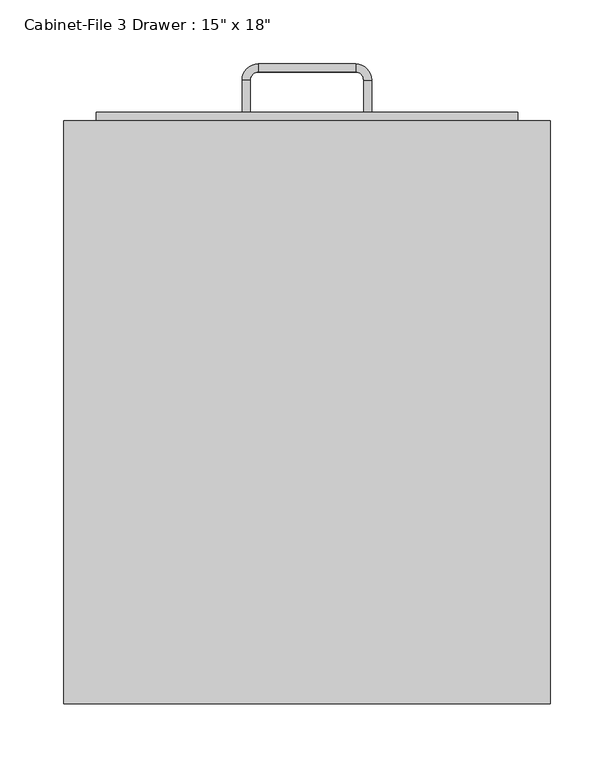
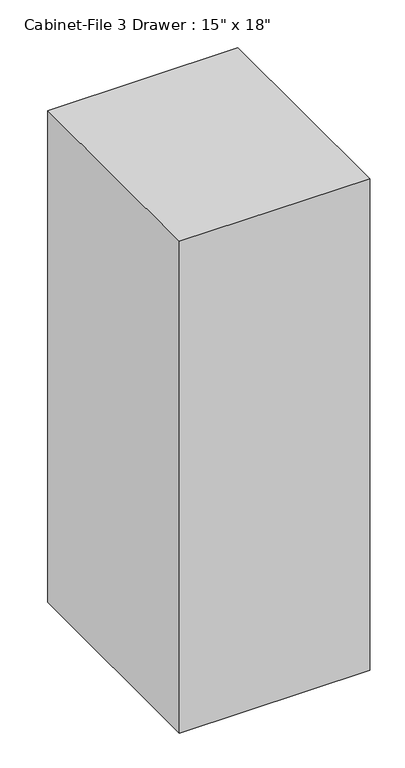
"""IFC4 building model written with IfcOpenShell, lengths in millimetres: furniture geometry."""

import ifcopenshell
import ifcopenshell.guid

model = None  # the IFC model being written
_history = None  # IfcOwnerHistory: only IFC2X3 demands one
_inside = {}  # id of a spatial element -> (the spatial element, [elements in it])
_under = {}  # id of a project, library or spatial element -> (it, [spatial elements below it])
_declared = {}  # id of a project -> (the project, [libraries it declares])
_typed = {}  # id of a type object -> (the type object, [elements of that type])
_made_of = {}  # id of a material, layer set ... -> (it, [elements and type objects made of it])


def new_model(schema):
    """Start an empty IFC model of exactly this schema.

    Asked for "IFC4X3", IfcOpenShell would pick the latest addendum, in which some entities
    have other attributes; the version numbers below select the first issue.
    IFC2X3 requires an IfcOwnerHistory on every rooted entity: one is made here for all.
    """
    global model, _history
    if schema == "IFC4X3":
        model = ifcopenshell.file(schema_version=(4, 3, 0, 0))
    else:
        model = ifcopenshell.file(schema=schema)
    _inside.clear()
    _under.clear()
    _declared.clear()
    _typed.clear()
    _made_of.clear()
    _history = None
    if model.schema == "IFC2X3":
        org = make("IfcOrganization", Name="unknown")
        user = make(
            "IfcPersonAndOrganization",
            ThePerson=make("IfcPerson", FamilyName="unknown"),
            TheOrganization=org,
        )
        app = make(
            "IfcApplication",
            ApplicationDeveloper=org,
            Version="unknown",
            ApplicationFullName="unknown",
            ApplicationIdentifier="unknown",
        )
        _history = make(
            "IfcOwnerHistory",
            OwningUser=user,
            OwningApplication=app,
            ChangeAction="ADDED",
            CreationDate=0,
        )
    return model


def make(cls, **values):
    """One entity of the class cls with the attributes given. An attribute that is None is left unset."""
    return model.create_entity(
        cls, **{name: value for name, value in values.items() if value is not None}
    )


def rooted(cls, **values):
    """An entity with a GlobalId (a new one), such as an element, a storey or a relation."""
    return make(cls, GlobalId=ifcopenshell.guid.new(), OwnerHistory=_history, **values)


def si_unit(unit_type, name, prefix=None):
    """IfcSIUnit, for example si_unit("LENGTHUNIT", "METRE", prefix="MILLI")."""
    return make("IfcSIUnit", UnitType=unit_type, Prefix=prefix, Name=name)


def assignment(units):
    """IfcUnitAssignment: the units of a project."""
    return None if units is None else make("IfcUnitAssignment", Units=units)


def point(xyz):
    """IfcCartesianPoint."""
    return None if xyz is None else make("IfcCartesianPoint", Coordinates=xyz)


def direction(xyz):
    """IfcDirection."""
    return None if xyz is None else make("IfcDirection", DirectionRatios=xyz)


def frame(location, z_axis=None, x_axis=None):
    """IfcAxis2Placement3D, a coordinate frame: its origin and axes. An axis left out is left unset."""
    return make(
        "IfcAxis2Placement3D",
        Location=point(location),
        Axis=direction(z_axis),
        RefDirection=direction(x_axis),
    )


def origin():
    """The frame at (0, 0, 0) with its axes left unset."""
    return frame((0.0, 0.0, 0.0))


def origin_with_axes():
    """The frame at (0, 0, 0) with the z axis (0, 0, 1) and the x axis (1, 0, 0) written out."""
    return frame((0.0, 0.0, 0.0), z_axis=(0.0, 0.0, 1.0), x_axis=(1.0, 0.0, 0.0))


def place(relative_to, where):
    """IfcLocalPlacement: puts the frame where relative to a parent placement (None: the world)."""
    return make(
        "IfcLocalPlacement", PlacementRelTo=relative_to, RelativePlacement=where
    )


def context(
    kind, dimensions, precision=None, world=None, true_north=None, identifier=None
):
    """IfcGeometricRepresentationContext, for example the 3D "Model" context."""
    return make(
        "IfcGeometricRepresentationContext",
        ContextIdentifier=identifier,
        ContextType=kind,
        CoordinateSpaceDimension=dimensions,
        Precision=precision,
        WorldCoordinateSystem=world,
        TrueNorth=true_north,
    )


def project(units=None, contexts=None):
    """IfcProject with its units and contexts."""
    return rooted(
        "IfcProject",
        Name="project",
        RepresentationContexts=contexts,
        UnitsInContext=assignment(units),
    )


def spatial(cls, under=None, at=None, **own):
    """A site, building, storey or space (cls), placed at a placement, below another one or the project."""
    s = rooted(cls, ObjectPlacement=at, **own)
    if under is not None:
        _under.setdefault(under.id(), (under, []))[1].append(s)
    return s


def polyline(points):
    """IfcPolyline through the points."""
    return make("IfcPolyline", Points=[point(p) for p in points])


def circle_curve(where, radius):
    """IfcCircle in the frame where."""
    return make("IfcCircle", Position=where, Radius=radius)


def outline(outer, holes=None, kind="AREA"):
    """IfcArbitraryClosedProfileDef: a profile drawn as a closed curve; with holes, ...WithVoids."""
    if holes is None:
        return make("IfcArbitraryClosedProfileDef", ProfileType=kind, OuterCurve=outer)
    return make(
        "IfcArbitraryProfileDefWithVoids",
        ProfileType=kind,
        OuterCurve=outer,
        InnerCurves=holes,
    )


def extrude(swept, where, along, depth):
    """IfcExtrudedAreaSolid: the profile swept, set in the frame where, extruded along a direction by depth."""
    return make(
        "IfcExtrudedAreaSolid",
        SweptArea=swept,
        Position=where,
        ExtrudedDirection=direction(along),
        Depth=depth,
    )


def shape(context_of_items, identifier, shape_type, items):
    """IfcShapeRepresentation: the items that make up one representation, for example the "Body"."""
    return make(
        "IfcShapeRepresentation",
        ContextOfItems=context_of_items,
        RepresentationIdentifier=identifier,
        RepresentationType=shape_type,
        Items=items,
    )


def source(mapping_origin, context_of_items, identifier, shape_type, items):
    """IfcRepresentationMap: a shape defined once, which mapped items show again and again."""
    return make(
        "IfcRepresentationMap",
        MappingOrigin=mapping_origin,
        MappedRepresentation=shape(context_of_items, identifier, shape_type, items),
    )


def transform(
    local_origin,
    x_axis=None,
    y_axis=None,
    z_axis=None,
    scale=None,
    scale2=None,
    scale3=None,
    uniform=True,
):
    """IfcCartesianTransformationOperator3D, or its non-uniform kind. x_axis, y_axis, z_axis: its Axis1, 2, 3."""
    if uniform:
        return make(
            "IfcCartesianTransformationOperator3D",
            Axis1=direction(x_axis),
            Axis2=direction(y_axis),
            LocalOrigin=point(local_origin),
            Scale=scale,
            Axis3=direction(z_axis),
        )
    return make(
        "IfcCartesianTransformationOperator3DnonUniform",
        Axis1=direction(x_axis),
        Axis2=direction(y_axis),
        LocalOrigin=point(local_origin),
        Scale=scale,
        Axis3=direction(z_axis),
        Scale2=scale2,
        Scale3=scale3,
    )


def mapped(mapping_source, mapping_target):
    """IfcMappedItem: shows the shape of a source again, moved by a transform."""
    return make(
        "IfcMappedItem", MappingSource=mapping_source, MappingTarget=mapping_target
    )


def made_of(thing, what):
    """Note that an element or type object is made of a material, layer set ...; save() writes the relation."""
    if what is not None:
        _made_of.setdefault(what.id(), (what, []))[1].append(thing)
    return thing


def element(
    cls,
    number,
    at=None,
    inside=None,
    cuts=None,
    type_object=None,
    material=None,
    context=None,
    identifier="Body",
    shape_type=None,
    held_by="IfcProductDefinitionShape",
    body=None,
    shapes=None,
    **own,
):
    """One element of the class cls, such as IfcWall. Its Tag is "e" and its number.

    at: its placement. inside: the storey or other place that contains it. cuts: it is an
    opening in that element (IfcRelVoidsElement). A single representation is given by context,
    identifier, shape_type and body (its items); several are given by shapes. held_by: the class
    of the entity that holds the representations. save() writes the other relations.
    """
    e = rooted(cls, Tag="e%d" % number, ObjectPlacement=at, **own)
    if body is not None:
        shapes = [shape(context, identifier, shape_type, body)]
    if shapes is not None:
        e.Representation = make(held_by, Representations=shapes)
    if inside is not None:
        _inside.setdefault(inside.id(), (inside, []))[1].append(e)
    if cuts is not None:
        rooted(
            "IfcRelVoidsElement", RelatingBuildingElement=cuts, RelatedOpeningElement=e
        )
    if type_object is not None:
        _typed.setdefault(type_object.id(), (type_object, []))[1].append(e)
    return made_of(e, material)


def aggregate(whole, parts):
    """IfcRelAggregates: a whole, such as a stair, and the parts it consists of."""
    return rooted("IfcRelAggregates", RelatingObject=whole, RelatedObjects=parts)


def save(model, path):
    """Write the relations noted so far, then the file.

    IfcRelAggregates (storeys below a building ...), IfcRelContainedInSpatialStructure (elements
    in a storey), IfcRelDefinesByType, IfcRelAssociatesMaterial and IfcRelDeclares: one each for
    every whole, place, type object, material and project.
    """
    for whole, parts in _under.values():
        aggregate(whole, parts)
    for where, things in _inside.values():
        rooted(
            "IfcRelContainedInSpatialStructure",
            RelatedElements=things,
            RelatingStructure=where,
        )
    for kind, things in _typed.values():
        rooted("IfcRelDefinesByType", RelatedObjects=things, RelatingType=kind)
    for what, things in _made_of.values():
        rooted("IfcRelAssociatesMaterial", RelatedObjects=things, RelatingMaterial=what)
    for by, libraries in _declared.values():
        rooted("IfcRelDeclares", RelatingContext=by, RelatedDefinitions=libraries)
    model.write(path)


def plane_surface(at):
    """IfcPlane: the flat surface through the origin of the frame at, square to its z axis."""
    return make("IfcPlane", Position=at)


def cylinder_surface(at, radius):
    """IfcCylindricalSurface: all points at the distance radius from the z axis of the frame at."""
    return make("IfcCylindricalSurface", Position=at, Radius=radius)


def revolved_surface(curve, axis_point, axis_direction):
    """IfcSurfaceOfRevolution: the curve turned about the line through axis_point along axis_direction."""
    return make(
        "IfcSurfaceOfRevolution",
        SweptCurve=make("IfcArbitraryOpenProfileDef", ProfileType="CURVE", Curve=curve),
        AxisPosition=make("IfcAxis1Placement", Location=point(axis_point), Axis=direction(axis_direction)),
    )


def advanced_brep(points, edges, surfaces, faces):
    """IfcAdvancedBrep: a solid bounded by faces that lie on surfaces and meet in shared edges.

    An edge is (start, end): straight between two places in points (the first is 0);
    or (start, end, curve); or (start, end, curve, False) where it runs against its curve.
    A face is (place in surfaces, loops), or (place, loops, False) where it looks against
    its surface's normal. A loop lists edges by number (the first is 1), with a minus sign
    where the edge is run from its end to its start. The first loop is the outer one.
    """
    corners = [point(p) for p in points]
    vertices = [make("IfcVertexPoint", VertexGeometry=c) for c in corners]
    made = []
    for start, end, *more in edges:
        made.append(
            make(
                "IfcEdgeCurve",
                EdgeStart=vertices[start],
                EdgeEnd=vertices[end],
                EdgeGeometry=more[0] if more else make("IfcPolyline", Points=[corners[start], corners[end]]),
                SameSense=more[1] if len(more) > 1 else True,
            )
        )
    hull = []
    for where, loops, *sense in faces:
        bounds = []
        for j, loop in enumerate(loops):
            ring = [make("IfcOrientedEdge", EdgeElement=made[abs(k) - 1], Orientation=k > 0) for k in loop]
            bounds.append(
                make(
                    "IfcFaceOuterBound" if j == 0 else "IfcFaceBound",
                    Bound=make("IfcEdgeLoop", EdgeList=ring),
                    Orientation=True,
                )
            )
        hull.append(make("IfcAdvancedFace", Bounds=bounds, FaceSurface=surfaces[where], SameSense=sense[0] if sense else True))
    return make("IfcAdvancedBrep", Outer=make("IfcClosedShell", CfsFaces=hull))


def furniture_48aa8ab9(model_context):
    return source(origin(), model_context, "Body", "SolidModel", [
        extrude(outline(polyline([(62.603553, -86.4656999), (-318.396447, -86.4656999), (-318.396447, 370.7343001), (62.603553, 370.7343001), (62.603553, -86.4656999)])), origin_with_axes(), (0.0, 0.0, 1.0), 1041.4),
        extrude(outline(polyline([(37.203553, 377.0843001), (37.203553, 370.7343001), (-292.996447, 370.7343001), (-292.996447, 377.0843001), (37.203553, 377.0843001)])), frame((0.0, 0.0, 736.6), z_axis=(0.0, 0.0, 1.0), x_axis=(1.0, 0.0, 0.0)), (0.0, 0.0, 1.0), 279.4),
        extrude(outline(polyline([(37.203553, 377.0843001), (37.203553, 370.7343001), (-292.996447, 370.7343001), (-292.996447, 377.0843001), (37.203553, 377.0843001)])), frame((0.0, 0.0, 431.8), z_axis=(0.0, 0.0, 1.0), x_axis=(1.0, 0.0, 0.0)), (0.0, 0.0, 1.0), 279.4),
        extrude(outline(polyline([(37.203553, 377.0843001), (37.203553, 370.7343001), (-292.996447, 370.7343001), (-292.996447, 377.0843001), (37.203553, 377.0843001)])), frame((0.0, 0.0, 127.0), z_axis=(0.0, 0.0, 1.0), x_axis=(1.0, 0.0, 0.0)), (0.0, 0.0, 1.0), 279.4),
        advanced_brep(
        [(-172.346447, 377.0843001, 203.2), (-172.346447, 377.0843001, 215.9), (-178.696447, 377.0843001, 215.9), (-178.696447, 377.0843001, 203.2), (-178.696447, 402.4843001, 203.2), (-172.346447, 402.4843001, 203.2), (-178.696447, 402.4843001, 215.9), (-172.346447, 402.4843001, 215.9), (-165.996447, 415.1843001, 203.2), (-165.996447, 408.8343001, 203.2), (-165.996447, 415.1843001, 215.9), (-165.996447, 408.8343001, 215.9), (-89.796447, 415.1843001, 203.2), (-89.796447, 408.8343001, 203.2), (-89.796447, 415.1843001, 215.9), (-89.796447, 408.8343001, 215.9), (-77.096447, 402.4843001, 203.2), (-83.446447, 402.4843001, 203.2), (-77.096447, 402.4843001, 215.9), (-83.446447, 402.4843001, 215.9), (-83.446447, 377.0843001, 203.2), (-77.096447, 377.0843001, 203.2), (-77.096447, 377.0843001, 215.9), (-83.446447, 377.0843001, 215.9)],
        [
            (0, 1),
            (1, 2),
            (2, 3),
            (3, 0),
            (3, 4),
            (4, 5),
            (5, 0),
            (2, 6),
            (6, 4),
            (1, 7),
            (7, 6),
            (5, 7),
            (8, 9),
            (9, 5, circle_curve(frame((-165.996447, 402.4843001, 203.2), z_axis=(0.0, 0.0, 1.0), x_axis=(-1.0, 0.0, 0.0)), 6.35)),
            (4, 8, circle_curve(frame((-165.996447, 402.4843001, 203.2), z_axis=(0.0, 0.0, -1.0), x_axis=(-1.0, 0.0, 0.0)), 12.7)),
            (10, 8),
            (6, 10, circle_curve(frame((-165.996447, 402.4843001, 215.9), z_axis=(0.0, 0.0, -1.0), x_axis=(-1.0, 0.0, 0.0)), 12.7)),
            (11, 10),
            (7, 11, circle_curve(frame((-165.996447, 402.4843001, 215.9), z_axis=(0.0, 0.0, -1.0), x_axis=(-1.0, 0.0, 0.0)), 6.35)),
            (9, 11),
            (8, 12),
            (12, 13),
            (13, 9),
            (10, 14),
            (14, 12),
            (11, 15),
            (15, 14),
            (13, 15),
            (16, 17),
            (17, 13, circle_curve(frame((-89.796447, 402.4843001, 203.2), z_axis=(0.0, 0.0, 1.0), x_axis=(0.0, 1.0, 0.0)), 6.35)),
            (12, 16, circle_curve(frame((-89.796447, 402.4843001, 203.2), z_axis=(0.0, 0.0, -1.0), x_axis=(0.0, 1.0, 0.0)), 12.7)),
            (18, 16),
            (14, 18, circle_curve(frame((-89.796447, 402.4843001, 215.9), z_axis=(0.0, 0.0, -1.0), x_axis=(0.0, 1.0, 0.0)), 12.7)),
            (19, 18),
            (15, 19, circle_curve(frame((-89.796447, 402.4843001, 215.9), z_axis=(0.0, 0.0, -1.0), x_axis=(0.0, 1.0, 0.0)), 6.35)),
            (17, 19),
            (20, 21),
            (21, 22),
            (22, 23),
            (23, 20),
            (16, 21),
            (20, 17),
            (18, 22),
            (19, 23),
        ],
        [
            plane_surface(frame((-978.8216451, 377.0843001, 0.0), z_axis=(0.0, -1.0, 0.0), x_axis=(0.0, 0.0, -1.0))),
            plane_surface(frame((-172.346447, 377.0843001, 203.2), z_axis=(0.0, 0.0, -1.0), x_axis=(0.0, 1.0, 0.0))),
            plane_surface(frame((-178.696447, 377.0843001, 203.2), z_axis=(-1.0, 0.0, 0.0), x_axis=(0.0, 1.0, 0.0))),
            plane_surface(frame((-178.696447, 377.0843001, 215.9), z_axis=(0.0, 0.0, 1.0), x_axis=(0.0, 1.0, 0.0))),
            plane_surface(frame((-172.346447, 377.0843001, 215.9), z_axis=(1.0, 0.0, 0.0), x_axis=(0.0, 1.0, 0.0))),
            plane_surface(frame((-165.996447, 402.4843001, 203.2), z_axis=(0.0, 0.0, -1.0), x_axis=(-1.0, 0.0, 0.0))),
            cylinder_surface(frame((-165.996447, 402.4843001, 0.0), z_axis=(0.0, 0.0, 1.0), x_axis=(-1.0, 0.0, 0.0)), 12.7),
            plane_surface(frame((-165.996447, 402.4843001, 215.9), z_axis=(0.0, 0.0, 1.0), x_axis=(-1.0, 0.0, 0.0))),
            revolved_surface(polyline([(-172.34644699999998, 402.4843001, 215.9), (-172.34644699999998, 402.4843001, 203.2)]), (-165.996447, 402.4843001, 0.0), (0.0, 0.0, 1.0)),
            plane_surface(frame((-165.996447, 408.8343001, 203.2), z_axis=(0.0, 0.0, -1.0), x_axis=(1.0, 0.0, 0.0))),
            plane_surface(frame((-165.996447, 415.1843001, 203.2), z_axis=(0.0, 1.0, 0.0), x_axis=(1.0, 0.0, 0.0))),
            plane_surface(frame((-165.996447, 415.1843001, 215.9), z_axis=(0.0, 0.0, 1.0), x_axis=(1.0, 0.0, 0.0))),
            plane_surface(frame((-165.996447, 408.8343001, 215.9), z_axis=(0.0, -1.0, 0.0), x_axis=(1.0, 0.0, 0.0))),
            plane_surface(frame((-89.796447, 402.4843001, 203.2), z_axis=(0.0, 0.0, -1.0), x_axis=(0.0, 1.0, 0.0))),
            cylinder_surface(frame((-89.796447, 402.4843001, 0.0), z_axis=(0.0, 0.0, 1.0), x_axis=(0.0, 1.0, 0.0)), 12.7),
            plane_surface(frame((-89.796447, 402.4843001, 215.9), z_axis=(0.0, 0.0, 1.0), x_axis=(0.0, 1.0, 0.0))),
            revolved_surface(polyline([(-89.796447, 408.8343001, 215.9), (-89.796447, 408.8343001, 203.2)]), (-89.796447, 402.4843001, 0.0), (0.0, 0.0, 1.0)),
            plane_surface(frame((-877.2216451, 377.0843001, 0.0), z_axis=(0.0, -1.0, 0.0), x_axis=(0.0, 0.0, 1.0))),
            plane_surface(frame((-83.446447, 402.4843001, 203.2), z_axis=(0.0, 0.0, -1.0), x_axis=(0.0, -1.0, 0.0))),
            plane_surface(frame((-77.096447, 402.4843001, 203.2), z_axis=(1.0, 0.0, 0.0), x_axis=(0.0, -1.0, 0.0))),
            plane_surface(frame((-77.096447, 402.4843001, 215.9), z_axis=(0.0, 0.0, 1.0), x_axis=(0.0, -1.0, 0.0))),
            plane_surface(frame((-83.446447, 402.4843001, 215.9), z_axis=(-1.0, 0.0, 0.0), x_axis=(0.0, -1.0, 0.0))),
        ],
        [
            (0, [[1, 2, 3, 4]]),
            (1, [[5, 6, 7, -4]]),
            (2, [[8, 9, -5, -3]]),
            (3, [[10, 11, -8, -2]]),
            (4, [[-7, 12, -10, -1]]),
            (5, [[13, 14, -6, 15]]),
            (6, [[16, -15, -9, 17]]),
            (7, [[18, -17, -11, 19]]),
            (8, [[20, -19, -12, -14]]),
            (9, [[21, 22, 23, -13]]),
            (10, [[24, 25, -21, -16]]),
            (11, [[26, 27, -24, -18]]),
            (12, [[-23, 28, -26, -20]]),
            (13, [[29, 30, -22, 31]]),
            (14, [[32, -31, -25, 33]]),
            (15, [[34, -33, -27, 35]]),
            (16, [[36, -35, -28, -30]]),
            (17, [[37, 38, 39, 40]]),
            (18, [[41, -37, 42, -29]]),
            (19, [[43, -38, -41, -32]]),
            (20, [[44, -39, -43, -34]]),
            (21, [[-42, -40, -44, -36]]),
        ],
    ),
        advanced_brep(
        [(-172.346447, 377.0843001, 482.6), (-172.346447, 377.0843001, 495.3), (-178.696447, 377.0843001, 495.3), (-178.696447, 377.0843001, 482.6), (-178.696447, 402.4843001, 482.6), (-172.346447, 402.4843001, 482.6), (-178.696447, 402.4843001, 495.3), (-172.346447, 402.4843001, 495.3), (-165.996447, 415.1843001, 482.6), (-165.996447, 408.8343001, 482.6), (-165.996447, 415.1843001, 495.3), (-165.996447, 408.8343001, 495.3), (-89.796447, 415.1843001, 482.6), (-89.796447, 408.8343001, 482.6), (-89.796447, 415.1843001, 495.3), (-89.796447, 408.8343001, 495.3), (-77.096447, 402.4843001, 482.6), (-83.446447, 402.4843001, 482.6), (-77.096447, 402.4843001, 495.3), (-83.446447, 402.4843001, 495.3), (-83.446447, 377.0843001, 482.6), (-77.096447, 377.0843001, 482.6), (-77.096447, 377.0843001, 495.3), (-83.446447, 377.0843001, 495.3)],
        [
            (0, 1),
            (1, 2),
            (2, 3),
            (3, 0),
            (3, 4),
            (4, 5),
            (5, 0),
            (2, 6),
            (6, 4),
            (1, 7),
            (7, 6),
            (5, 7),
            (8, 9),
            (9, 5, circle_curve(frame((-165.996447, 402.4843001, 482.6), z_axis=(0.0, 0.0, 1.0), x_axis=(-1.0, 0.0, 0.0)), 6.35)),
            (4, 8, circle_curve(frame((-165.996447, 402.4843001, 482.6), z_axis=(0.0, 0.0, -1.0), x_axis=(-1.0, 0.0, 0.0)), 12.7)),
            (10, 8),
            (6, 10, circle_curve(frame((-165.996447, 402.4843001, 495.3), z_axis=(0.0, 0.0, -1.0), x_axis=(-1.0, 0.0, 0.0)), 12.7)),
            (11, 10),
            (7, 11, circle_curve(frame((-165.996447, 402.4843001, 495.3), z_axis=(0.0, 0.0, -1.0), x_axis=(-1.0, 0.0, 0.0)), 6.35)),
            (9, 11),
            (8, 12),
            (12, 13),
            (13, 9),
            (10, 14),
            (14, 12),
            (11, 15),
            (15, 14),
            (13, 15),
            (16, 17),
            (17, 13, circle_curve(frame((-89.796447, 402.4843001, 482.6), z_axis=(0.0, 0.0, 1.0), x_axis=(0.0, 1.0, 0.0)), 6.35)),
            (12, 16, circle_curve(frame((-89.796447, 402.4843001, 482.6), z_axis=(0.0, 0.0, -1.0), x_axis=(0.0, 1.0, 0.0)), 12.7)),
            (18, 16),
            (14, 18, circle_curve(frame((-89.796447, 402.4843001, 495.3), z_axis=(0.0, 0.0, -1.0), x_axis=(0.0, 1.0, 0.0)), 12.7)),
            (19, 18),
            (15, 19, circle_curve(frame((-89.796447, 402.4843001, 495.3), z_axis=(0.0, 0.0, -1.0), x_axis=(0.0, 1.0, 0.0)), 6.35)),
            (17, 19),
            (20, 21),
            (21, 22),
            (22, 23),
            (23, 20),
            (16, 21),
            (20, 17),
            (18, 22),
            (19, 23),
        ],
        [
            plane_surface(frame((-978.8216451, 377.0843001, 0.0), z_axis=(0.0, -1.0, 0.0), x_axis=(0.0, 0.0, -1.0))),
            plane_surface(frame((-172.346447, 377.0843001, 482.6), z_axis=(0.0, 0.0, -1.0), x_axis=(0.0, 1.0, 0.0))),
            plane_surface(frame((-178.696447, 377.0843001, 482.6), z_axis=(-1.0, 0.0, 0.0), x_axis=(0.0, 1.0, 0.0))),
            plane_surface(frame((-178.696447, 377.0843001, 495.3), z_axis=(0.0, 0.0, 1.0), x_axis=(0.0, 1.0, 0.0))),
            plane_surface(frame((-172.346447, 377.0843001, 495.3), z_axis=(1.0, 0.0, 0.0), x_axis=(0.0, 1.0, 0.0))),
            plane_surface(frame((-165.996447, 402.4843001, 482.6), z_axis=(0.0, 0.0, -1.0), x_axis=(-1.0, 0.0, 0.0))),
            cylinder_surface(frame((-165.996447, 402.4843001, 0.0), z_axis=(0.0, 0.0, 1.0), x_axis=(-1.0, 0.0, 0.0)), 12.7),
            plane_surface(frame((-165.996447, 402.4843001, 495.3), z_axis=(0.0, 0.0, 1.0), x_axis=(-1.0, 0.0, 0.0))),
            revolved_surface(polyline([(-172.34644699999998, 402.4843001, 495.3), (-172.34644699999998, 402.4843001, 482.6)]), (-165.996447, 402.4843001, 0.0), (0.0, 0.0, 1.0)),
            plane_surface(frame((-165.996447, 408.8343001, 482.6), z_axis=(0.0, 0.0, -1.0), x_axis=(1.0, 0.0, 0.0))),
            plane_surface(frame((-165.996447, 415.1843001, 482.6), z_axis=(0.0, 1.0, 0.0), x_axis=(1.0, 0.0, 0.0))),
            plane_surface(frame((-165.996447, 415.1843001, 495.3), z_axis=(0.0, 0.0, 1.0), x_axis=(1.0, 0.0, 0.0))),
            plane_surface(frame((-165.996447, 408.8343001, 495.3), z_axis=(0.0, -1.0, 0.0), x_axis=(1.0, 0.0, 0.0))),
            plane_surface(frame((-89.796447, 402.4843001, 482.6), z_axis=(0.0, 0.0, -1.0), x_axis=(0.0, 1.0, 0.0))),
            cylinder_surface(frame((-89.796447, 402.4843001, 0.0), z_axis=(0.0, 0.0, 1.0), x_axis=(0.0, 1.0, 0.0)), 12.7),
            plane_surface(frame((-89.796447, 402.4843001, 495.3), z_axis=(0.0, 0.0, 1.0), x_axis=(0.0, 1.0, 0.0))),
            revolved_surface(polyline([(-89.796447, 408.8343001, 495.3), (-89.796447, 408.8343001, 482.6)]), (-89.796447, 402.4843001, 0.0), (0.0, 0.0, 1.0)),
            plane_surface(frame((-877.2216451, 377.0843001, 0.0), z_axis=(0.0, -1.0, 0.0), x_axis=(0.0, 0.0, 1.0))),
            plane_surface(frame((-83.446447, 402.4843001, 482.6), z_axis=(0.0, 0.0, -1.0), x_axis=(0.0, -1.0, 0.0))),
            plane_surface(frame((-77.096447, 402.4843001, 482.6), z_axis=(1.0, 0.0, 0.0), x_axis=(0.0, -1.0, 0.0))),
            plane_surface(frame((-77.096447, 402.4843001, 495.3), z_axis=(0.0, 0.0, 1.0), x_axis=(0.0, -1.0, 0.0))),
            plane_surface(frame((-83.446447, 402.4843001, 495.3), z_axis=(-1.0, 0.0, 0.0), x_axis=(0.0, -1.0, 0.0))),
        ],
        [
            (0, [[1, 2, 3, 4]]),
            (1, [[5, 6, 7, -4]]),
            (2, [[8, 9, -5, -3]]),
            (3, [[10, 11, -8, -2]]),
            (4, [[-7, 12, -10, -1]]),
            (5, [[13, 14, -6, 15]]),
            (6, [[16, -15, -9, 17]]),
            (7, [[18, -17, -11, 19]]),
            (8, [[20, -19, -12, -14]]),
            (9, [[21, 22, 23, -13]]),
            (10, [[24, 25, -21, -16]]),
            (11, [[26, 27, -24, -18]]),
            (12, [[-23, 28, -26, -20]]),
            (13, [[29, 30, -22, 31]]),
            (14, [[32, -31, -25, 33]]),
            (15, [[34, -33, -27, 35]]),
            (16, [[36, -35, -28, -30]]),
            (17, [[37, 38, 39, 40]]),
            (18, [[41, -37, 42, -29]]),
            (19, [[43, -38, -41, -32]]),
            (20, [[44, -39, -43, -34]]),
            (21, [[-42, -40, -44, -36]]),
        ],
    ),
        advanced_brep(
        [(-172.346447, 377.0843001, 787.4), (-172.346447, 377.0843001, 800.1), (-178.696447, 377.0843001, 800.1), (-178.696447, 377.0843001, 787.4), (-178.696447, 402.4843001, 787.4), (-172.346447, 402.4843001, 787.4), (-178.696447, 402.4843001, 800.1), (-172.346447, 402.4843001, 800.1), (-165.996447, 415.1843001, 787.4), (-165.996447, 408.8343001, 787.4), (-165.996447, 415.1843001, 800.1), (-165.996447, 408.8343001, 800.1), (-89.796447, 415.1843001, 787.4), (-89.796447, 408.8343001, 787.4), (-89.796447, 415.1843001, 800.1), (-89.796447, 408.8343001, 800.1), (-77.096447, 402.4843001, 787.4), (-83.446447, 402.4843001, 787.4), (-77.096447, 402.4843001, 800.1), (-83.446447, 402.4843001, 800.1), (-83.446447, 377.0843001, 787.4), (-77.096447, 377.0843001, 787.4), (-77.096447, 377.0843001, 800.1), (-83.446447, 377.0843001, 800.1)],
        [
            (0, 1),
            (1, 2),
            (2, 3),
            (3, 0),
            (3, 4),
            (4, 5),
            (5, 0),
            (2, 6),
            (6, 4),
            (1, 7),
            (7, 6),
            (5, 7),
            (8, 9),
            (9, 5, circle_curve(frame((-165.996447, 402.4843001, 787.4), z_axis=(0.0, 0.0, 1.0), x_axis=(-1.0, 0.0, 0.0)), 6.35)),
            (4, 8, circle_curve(frame((-165.996447, 402.4843001, 787.4), z_axis=(0.0, 0.0, -1.0), x_axis=(-1.0, 0.0, 0.0)), 12.7)),
            (10, 8),
            (6, 10, circle_curve(frame((-165.996447, 402.4843001, 800.1), z_axis=(0.0, 0.0, -1.0), x_axis=(-1.0, 0.0, 0.0)), 12.7)),
            (11, 10),
            (7, 11, circle_curve(frame((-165.996447, 402.4843001, 800.1), z_axis=(0.0, 0.0, -1.0), x_axis=(-1.0, 0.0, 0.0)), 6.35)),
            (9, 11),
            (8, 12),
            (12, 13),
            (13, 9),
            (10, 14),
            (14, 12),
            (11, 15),
            (15, 14),
            (13, 15),
            (16, 17),
            (17, 13, circle_curve(frame((-89.796447, 402.4843001, 787.4), z_axis=(0.0, 0.0, 1.0), x_axis=(0.0, 1.0, 0.0)), 6.35)),
            (12, 16, circle_curve(frame((-89.796447, 402.4843001, 787.4), z_axis=(0.0, 0.0, -1.0), x_axis=(0.0, 1.0, 0.0)), 12.7)),
            (18, 16),
            (14, 18, circle_curve(frame((-89.796447, 402.4843001, 800.1), z_axis=(0.0, 0.0, -1.0), x_axis=(0.0, 1.0, 0.0)), 12.7)),
            (19, 18),
            (15, 19, circle_curve(frame((-89.796447, 402.4843001, 800.1), z_axis=(0.0, 0.0, -1.0), x_axis=(0.0, 1.0, 0.0)), 6.35)),
            (17, 19),
            (20, 21),
            (21, 22),
            (22, 23),
            (23, 20),
            (16, 21),
            (20, 17),
            (18, 22),
            (19, 23),
        ],
        [
            plane_surface(frame((-978.8216451, 377.0843001, 0.0), z_axis=(0.0, -1.0, 0.0), x_axis=(0.0, 0.0, -1.0))),
            plane_surface(frame((-172.346447, 377.0843001, 787.4), z_axis=(0.0, 0.0, -1.0), x_axis=(0.0, 1.0, 0.0))),
            plane_surface(frame((-178.696447, 377.0843001, 787.4), z_axis=(-1.0, 0.0, 0.0), x_axis=(0.0, 1.0, 0.0))),
            plane_surface(frame((-178.696447, 377.0843001, 800.1), z_axis=(0.0, 0.0, 1.0), x_axis=(0.0, 1.0, 0.0))),
            plane_surface(frame((-172.346447, 377.0843001, 800.1), z_axis=(1.0, 0.0, 0.0), x_axis=(0.0, 1.0, 0.0))),
            plane_surface(frame((-165.996447, 402.4843001, 787.4), z_axis=(0.0, 0.0, -1.0), x_axis=(-1.0, 0.0, 0.0))),
            cylinder_surface(frame((-165.996447, 402.4843001, 0.0), z_axis=(0.0, 0.0, 1.0), x_axis=(-1.0, 0.0, 0.0)), 12.7),
            plane_surface(frame((-165.996447, 402.4843001, 800.1), z_axis=(0.0, 0.0, 1.0), x_axis=(-1.0, 0.0, 0.0))),
            revolved_surface(polyline([(-172.34644699999998, 402.4843001, 800.1), (-172.34644699999998, 402.4843001, 787.4)]), (-165.996447, 402.4843001, 0.0), (0.0, 0.0, 1.0)),
            plane_surface(frame((-165.996447, 408.8343001, 787.4), z_axis=(0.0, 0.0, -1.0), x_axis=(1.0, 0.0, 0.0))),
            plane_surface(frame((-165.996447, 415.1843001, 787.4), z_axis=(0.0, 1.0, 0.0), x_axis=(1.0, 0.0, 0.0))),
            plane_surface(frame((-165.996447, 415.1843001, 800.1), z_axis=(0.0, 0.0, 1.0), x_axis=(1.0, 0.0, 0.0))),
            plane_surface(frame((-165.996447, 408.8343001, 800.1), z_axis=(0.0, -1.0, 0.0), x_axis=(1.0, 0.0, 0.0))),
            plane_surface(frame((-89.796447, 402.4843001, 787.4), z_axis=(0.0, 0.0, -1.0), x_axis=(0.0, 1.0, 0.0))),
            cylinder_surface(frame((-89.796447, 402.4843001, 0.0), z_axis=(0.0, 0.0, 1.0), x_axis=(0.0, 1.0, 0.0)), 12.7),
            plane_surface(frame((-89.796447, 402.4843001, 800.1), z_axis=(0.0, 0.0, 1.0), x_axis=(0.0, 1.0, 0.0))),
            revolved_surface(polyline([(-89.796447, 408.8343001, 800.1), (-89.796447, 408.8343001, 787.4)]), (-89.796447, 402.4843001, 0.0), (0.0, 0.0, 1.0)),
            plane_surface(frame((-877.2216451, 377.0843001, 0.0), z_axis=(0.0, -1.0, 0.0), x_axis=(0.0, 0.0, 1.0))),
            plane_surface(frame((-83.446447, 402.4843001, 787.4), z_axis=(0.0, 0.0, -1.0), x_axis=(0.0, -1.0, 0.0))),
            plane_surface(frame((-77.096447, 402.4843001, 787.4), z_axis=(1.0, 0.0, 0.0), x_axis=(0.0, -1.0, 0.0))),
            plane_surface(frame((-77.096447, 402.4843001, 800.1), z_axis=(0.0, 0.0, 1.0), x_axis=(0.0, -1.0, 0.0))),
            plane_surface(frame((-83.446447, 402.4843001, 800.1), z_axis=(-1.0, 0.0, 0.0), x_axis=(0.0, -1.0, 0.0))),
        ],
        [
            (0, [[1, 2, 3, 4]]),
            (1, [[5, 6, 7, -4]]),
            (2, [[8, 9, -5, -3]]),
            (3, [[10, 11, -8, -2]]),
            (4, [[-7, 12, -10, -1]]),
            (5, [[13, 14, -6, 15]]),
            (6, [[16, -15, -9, 17]]),
            (7, [[18, -17, -11, 19]]),
            (8, [[20, -19, -12, -14]]),
            (9, [[21, 22, 23, -13]]),
            (10, [[24, 25, -21, -16]]),
            (11, [[26, 27, -24, -18]]),
            (12, [[-23, 28, -26, -20]]),
            (13, [[29, 30, -22, 31]]),
            (14, [[32, -31, -25, 33]]),
            (15, [[34, -33, -27, 35]]),
            (16, [[36, -35, -28, -30]]),
            (17, [[37, 38, 39, 40]]),
            (18, [[41, -37, 42, -29]]),
            (19, [[43, -38, -41, -32]]),
            (20, [[44, -39, -43, -34]]),
            (21, [[-42, -40, -44, -36]]),
        ],
    ),
    ])


if __name__ == "__main__":
    model = new_model("IFC4")
    model_context = context("Model", 3, world=origin())
    ifc_project = project(units=[si_unit("LENGTHUNIT", "METRE", prefix="MILLI")], contexts=[model_context])
    site = spatial("IfcSite", under=ifc_project)
    building = spatial("IfcBuilding", under=site)
    placement = place(None, origin())
    furniture_shape = furniture_48aa8ab9(model_context)
    element("IfcFurniture", 1, ObjectType="Cabinet-File 3 Drawer : 15\" x 18\"", at=placement, inside=building, context=model_context, shape_type="MappedRepresentation", body=[
        mapped(furniture_shape, transform((0.0, 0.0, 0.0), x_axis=(1.0, 0.0, 0.0), y_axis=(0.0, 1.0, 0.0), z_axis=(0.0, 0.0, 1.0))),
    ])
    save(model, "model.ifc")

# Revit data of these elements
# Type "Cabinet-File 3 Drawer : 15\" x 18\""
#   Assembly Code = "E2020200"
#   Depth = 1' - 6"
#   Height = 3' - 5"
#   Width = 1' - 3"
#   Cabinet Material = Steel, Paint Finish, Ivory, Glossy
#   Handle Material = Steel, Chrome Plated
#   Default Elevation = 0
# Element 1 (IfcFurniture, "Cabinet-File 3 Drawer : 15\" x 18\"")
#   Materials on its faces: "Steel, Chrome Plated", "Steel, Paint Finish, Ivory, Glossy"
# Materials
#   "Steel, Paint Finish, Ivory, Glossy": class "Metal", colour RGB 247 247 239, transparency 0, Description = "Steel, paint finish, ivory, glossy", Cost = 0
#   "Steel, Chrome Plated": class "Metal", colour RGB 17 17 17, transparency 0, Description = "Chromiuim plated steel", Cost = 0
